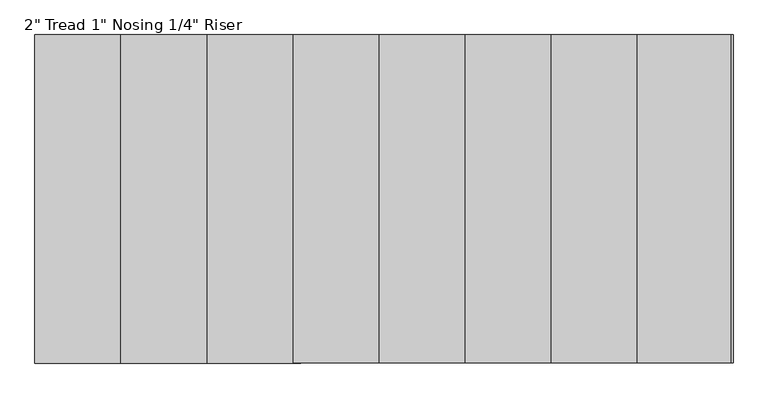
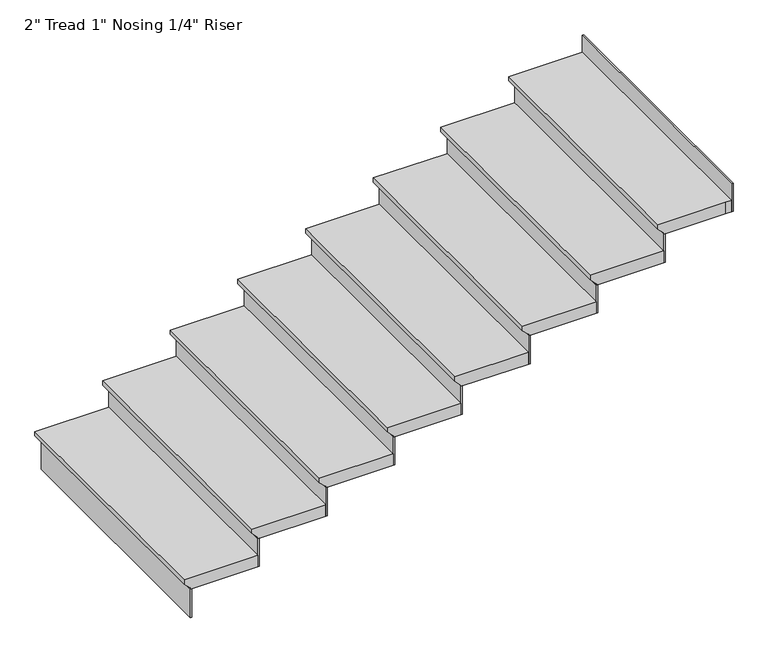
"""IFC4 building model written with IfcOpenShell, lengths in millimetres: stair flight geometry."""

from ifc_helpers import new_model, si_unit, origin, place, context, project, spatial, faceted_brep, source, transform, mapped, element, save


def stair_flight_4c000271(model_context):
    return source(origin(), model_context, "Body", "Brep", [
        faceted_brep([(663721.188677, -551651.2413841, 2328.7337838), (663721.188677, -551651.2413841, 2347.7837838), (663721.188677, -550584.4413841, 2347.7837838), (663721.188677, -550584.4413841, 2328.7337838), (663746.588677, -551651.2413841, 2303.3337838), (663746.588677, -550584.4413841, 2303.3337838), (664025.988677, -551651.2413841, 2347.7837838), (664025.988677, -550584.4413841, 2347.7837838), (663746.588677, -550584.4413841, 2296.9837838), (664025.988677, -550584.4413841, 2296.9837838), (664025.988677, -551651.2413841, 2296.9837838), (663746.588677, -551651.2413841, 2296.9837838)], [[[0, 1, 2, 3]], [[4, 0, 3, 5]], [[2, 1, 6, 7]], [[8, 9, 10, 11]], [[2, 7, 9, 8, 5, 3]], [[8, 11, 4, 5]], [[6, 1, 0, 4, 11, 10]], [[7, 6, 10, 9]]]),
        faceted_brep([(663746.588677, -551651.2413841, 2296.9837838), (663746.588677, -551651.2413841, 2173.4162162), (663752.938677, -551651.2413841, 2173.4162162), (663752.938677, -551651.2413841, 2296.9837838), (663746.588677, -550584.4413841, 2296.9837838), (663752.938677, -550584.4413841, 2296.9837838), (663752.938677, -550584.4413841, 2173.4162162), (663746.588677, -550584.4413841, 2173.4162162)], [[[0, 1, 2, 3]], [[4, 5, 6, 7]], [[1, 0, 4, 7]], [[2, 1, 7, 6]], [[3, 2, 6, 5]], [[0, 3, 5, 4]]]),
        faceted_brep([(664025.988677, -551651.2413841, 2420.5513514), (664025.988677, -551651.2413841, 2296.9837838), (664032.338677, -551651.2413841, 2296.9837838), (664032.338677, -551651.2413841, 2420.5513514), (664025.988677, -550584.4413841, 2420.5513514), (664032.338677, -550584.4413841, 2420.5513514), (664032.338677, -550584.4413841, 2296.9837838), (664025.988677, -550584.4413841, 2296.9837838)], [[[0, 1, 2, 3]], [[4, 5, 6, 7]], [[1, 0, 4, 7]], [[2, 1, 7, 6]], [[3, 2, 6, 5]], [[0, 3, 5, 4]]]),
        faceted_brep([(664000.588677, -550584.4413841, 2471.3513514), (664000.588677, -551651.2413841, 2471.3513514), (664305.388677, -551651.2413841, 2471.3513514), (664305.388677, -550584.4413841, 2471.3513514), (664025.988677, -550584.4413841, 2420.5513514), (664305.388677, -550584.4413841, 2420.5513514), (664305.388677, -551651.2413841, 2420.5513514), (664025.988677, -551651.2413841, 2420.5513514), (664025.988677, -550584.4413841, 2426.9013514), (664000.588677, -550584.4413841, 2452.3013514), (664025.988677, -551651.2413841, 2426.9013514), (664000.588677, -551651.2413841, 2452.3013514)], [[[0, 1, 2, 3]], [[4, 5, 6, 7]], [[0, 3, 5, 4, 8, 9]], [[4, 7, 10, 8]], [[2, 1, 11, 10, 7, 6]], [[3, 2, 6, 5]], [[11, 1, 0, 9]], [[10, 11, 9, 8]]]),
        faceted_brep([(664305.388677, -551651.2413841, 2544.1189189), (664305.388677, -551651.2413841, 2420.5513514), (664311.738677, -551651.2413841, 2420.5513514), (664311.738677, -551651.2413841, 2544.1189189), (664305.388677, -550584.4413841, 2544.1189189), (664311.738677, -550584.4413841, 2544.1189189), (664311.738677, -550584.4413841, 2420.5513514), (664305.388677, -550584.4413841, 2420.5513514)], [[[0, 1, 2, 3]], [[4, 5, 6, 7]], [[1, 0, 4, 7]], [[2, 1, 7, 6]], [[3, 2, 6, 5]], [[0, 3, 5, 4]]]),
        faceted_brep([(664279.988677, -550584.4413841, 2594.9189189), (664279.988677, -551651.2413841, 2594.9189189), (664584.788677, -551651.2413841, 2594.9189189), (664584.788677, -550584.4413841, 2594.9189189), (664305.388677, -550584.4413841, 2544.1189189), (664584.788677, -550584.4413841, 2544.1189189), (664584.788677, -551651.2413841, 2544.1189189), (664305.388677, -551651.2413841, 2544.1189189), (664305.388677, -550584.4413841, 2550.4689189), (664279.988677, -550584.4413841, 2575.8689189), (664305.388677, -551651.2413841, 2550.4689189), (664279.988677, -551651.2413841, 2575.8689189)], [[[0, 1, 2, 3]], [[4, 5, 6, 7]], [[0, 3, 5, 4, 8, 9]], [[4, 7, 10, 8]], [[2, 1, 11, 10, 7, 6]], [[3, 2, 6, 5]], [[11, 1, 0, 9]], [[10, 11, 9, 8]]]),
        faceted_brep([(664584.788677, -551651.2413841, 2667.6864865), (664584.788677, -551651.2413841, 2544.1189189), (664591.138677, -551651.2413841, 2544.1189189), (664591.138677, -551651.2413841, 2667.6864865), (664584.788677, -550584.4413841, 2667.6864865), (664591.138677, -550584.4413841, 2667.6864865), (664591.138677, -550584.4413841, 2544.1189189), (664584.788677, -550584.4413841, 2544.1189189)], [[[0, 1, 2, 3]], [[4, 5, 6, 7]], [[1, 0, 4, 7]], [[2, 1, 7, 6]], [[3, 2, 6, 5]], [[0, 3, 5, 4]]]),
        faceted_brep([(664559.388677, -550584.4413841, 2718.4864865), (664559.388677, -551651.2413841, 2718.4864865), (664864.188677, -551651.2413841, 2718.4864865), (664864.188677, -550584.4413841, 2718.4864865), (664584.788677, -550584.4413841, 2667.6864865), (664864.188677, -550584.4413841, 2667.6864865), (664864.188677, -551651.2413841, 2667.6864865), (664584.788677, -551651.2413841, 2667.6864865), (664584.788677, -550584.4413841, 2674.0364865), (664559.388677, -550584.4413841, 2699.4364865), (664584.788677, -551651.2413841, 2674.0364865), (664559.388677, -551651.2413841, 2699.4364865)], [[[0, 1, 2, 3]], [[4, 5, 6, 7]], [[0, 3, 5, 4, 8, 9]], [[4, 7, 10, 8]], [[2, 1, 11, 10, 7, 6]], [[3, 2, 6, 5]], [[11, 1, 0, 9]], [[10, 11, 9, 8]]]),
        faceted_brep([(664864.188677, -551651.2413841, 2791.2540541), (664864.188677, -551651.2413841, 2667.6864865), (664870.538677, -551651.2413841, 2667.6864865), (664870.538677, -551651.2413841, 2791.2540541), (664864.188677, -550584.4413841, 2791.2540541), (664870.538677, -550584.4413841, 2791.2540541), (664870.538677, -550584.4413841, 2667.6864865), (664864.188677, -550584.4413841, 2667.6864865)], [[[0, 1, 2, 3]], [[4, 5, 6, 7]], [[1, 0, 4, 7]], [[2, 1, 7, 6]], [[3, 2, 6, 5]], [[0, 3, 5, 4]]]),
        faceted_brep([(664838.788677, -550584.4413841, 2842.0540541), (664838.788677, -551651.2413841, 2842.0540541), (665143.588677, -551651.2413841, 2842.0540541), (665143.588677, -550584.4413841, 2842.0540541), (664864.188677, -550584.4413841, 2791.2540541), (665143.588677, -550584.4413841, 2791.2540541), (665143.588677, -551651.2413841, 2791.2540541), (664864.188677, -551651.2413841, 2791.2540541), (664864.188677, -550584.4413841, 2797.6040541), (664838.788677, -550584.4413841, 2823.0040541), (664864.188677, -551651.2413841, 2797.6040541), (664838.788677, -551651.2413841, 2823.0040541)], [[[0, 1, 2, 3]], [[4, 5, 6, 7]], [[0, 3, 5, 4, 8, 9]], [[4, 7, 10, 8]], [[2, 1, 11, 10, 7, 6]], [[3, 2, 6, 5]], [[11, 1, 0, 9]], [[10, 11, 9, 8]]]),
        faceted_brep([(665143.588677, -551651.2413841, 2914.8216216), (665143.588677, -551651.2413841, 2791.2540541), (665149.938677, -551651.2413841, 2791.2540541), (665149.938677, -551651.2413841, 2914.8216216), (665143.588677, -550584.4413841, 2914.8216216), (665149.938677, -550584.4413841, 2914.8216216), (665149.938677, -550584.4413841, 2791.2540541), (665143.588677, -550584.4413841, 2791.2540541)], [[[0, 1, 2, 3]], [[4, 5, 6, 7]], [[1, 0, 4, 7]], [[2, 1, 7, 6]], [[3, 2, 6, 5]], [[0, 3, 5, 4]]]),
        faceted_brep([(665118.188677, -550584.4413841, 2965.6216216), (665118.188677, -551651.2413841, 2965.6216216), (665422.988677, -551651.2413841, 2965.6216216), (665422.988677, -550584.4413841, 2965.6216216), (665143.588677, -550584.4413841, 2914.8216216), (665422.988677, -550584.4413841, 2914.8216216), (665422.988677, -551651.2413841, 2914.8216216), (665143.588677, -551651.2413841, 2914.8216216), (665143.588677, -550584.4413841, 2921.1716216), (665118.188677, -550584.4413841, 2946.5716216), (665143.588677, -551651.2413841, 2921.1716216), (665118.188677, -551651.2413841, 2946.5716216)], [[[0, 1, 2, 3]], [[4, 5, 6, 7]], [[0, 3, 5, 4, 8, 9]], [[4, 7, 10, 8]], [[2, 1, 11, 10, 7, 6]], [[3, 2, 6, 5]], [[11, 1, 0, 9]], [[10, 11, 9, 8]]]),
        faceted_brep([(665422.988677, -551651.2413841, 3038.3891892), (665422.988677, -551651.2413841, 2914.8216216), (665429.338677, -551651.2413841, 2914.8216216), (665429.338677, -551651.2413841, 3038.3891892), (665422.988677, -550584.4413841, 3038.3891892), (665429.338677, -550584.4413841, 3038.3891892), (665429.338677, -550584.4413841, 2914.8216216), (665422.988677, -550584.4413841, 2914.8216216)], [[[0, 1, 2, 3]], [[4, 5, 6, 7]], [[1, 0, 4, 7]], [[2, 1, 7, 6]], [[3, 2, 6, 5]], [[0, 3, 5, 4]]]),
        faceted_brep([(665397.588677, -550584.4413841, 3089.1891892), (665397.588677, -551651.2413841, 3089.1891892), (665702.388677, -551651.2413841, 3089.1891892), (665702.388677, -550584.4413841, 3089.1891892), (665422.988677, -550584.4413841, 3038.3891892), (665702.388677, -550584.4413841, 3038.3891892), (665702.388677, -551651.2413841, 3038.3891892), (665422.988677, -551651.2413841, 3038.3891892), (665422.988677, -550584.4413841, 3044.7391892), (665397.588677, -550584.4413841, 3070.1391892), (665422.988677, -551651.2413841, 3044.7391892), (665397.588677, -551651.2413841, 3070.1391892)], [[[0, 1, 2, 3]], [[4, 5, 6, 7]], [[0, 3, 5, 4, 8, 9]], [[4, 7, 10, 8]], [[2, 1, 11, 10, 7, 6]], [[3, 2, 6, 5]], [[11, 1, 0, 9]], [[10, 11, 9, 8]]]),
        faceted_brep([(665981.788677, -551651.2413841, 3285.5243243), (665981.788677, -551651.2413841, 3161.9567568), (665988.138677, -551651.2413841, 3161.9567568), (665988.138677, -551651.2413841, 3285.5243243), (665981.788677, -550584.4413841, 3285.5243243), (665988.138677, -550584.4413841, 3285.5243243), (665988.138677, -550584.4413841, 3161.9567568), (665981.788677, -550584.4413841, 3161.9567568)], [[[0, 1, 2, 3]], [[4, 5, 6, 7]], [[1, 0, 4, 7]], [[2, 1, 7, 6]], [[3, 2, 6, 5]], [[0, 3, 5, 4]]]),
        faceted_brep([(665702.388677, -551651.2413841, 3161.9567568), (665702.388677, -551651.2413841, 3038.3891892), (665708.738677, -551651.2413841, 3038.3891892), (665708.738677, -551651.2413841, 3161.9567568), (665702.388677, -550584.4413841, 3161.9567568), (665708.738677, -550584.4413841, 3161.9567568), (665708.738677, -550584.4413841, 3038.3891892), (665702.388677, -550584.4413841, 3038.3891892)], [[[0, 1, 2, 3]], [[4, 5, 6, 7]], [[1, 0, 4, 7]], [[2, 1, 7, 6]], [[3, 2, 6, 5]], [[0, 3, 5, 4]]]),
        faceted_brep([(665676.988677, -550584.4413841, 3212.7567568), (665676.988677, -551651.2413841, 3212.7567568), (665956.388677, -551651.2413841, 3212.7567568), (665981.788677, -551651.2413841, 3212.7567568), (665981.788677, -550584.4413841, 3212.7567568), (665702.388677, -550584.4413841, 3161.9567568), (665981.788677, -550584.4413841, 3161.9567568), (665981.788677, -551651.2413841, 3161.9567568), (665956.388677, -551651.2413841, 3161.9567568), (665702.388677, -551651.2413841, 3161.9567568), (665702.388677, -550584.4413841, 3168.3067568), (665676.988677, -550584.4413841, 3193.7067568), (665702.388677, -551651.2413841, 3168.3067568), (665676.988677, -551651.2413841, 3193.7067568)], [[[0, 1, 2, 3, 4]], [[5, 6, 7, 8, 9]], [[0, 4, 6, 5, 10, 11]], [[5, 9, 12, 10]], [[2, 1, 13, 12, 9, 8]], [[3, 2, 8, 7]], [[4, 3, 7, 6]], [[13, 1, 0, 11]], [[12, 13, 11, 10]]]),
    ])


if __name__ == "__main__":
    model = new_model("IFC4")
    model_context = context("Model", 3, world=origin())
    ifc_project = project(units=[si_unit("LENGTHUNIT", "METRE", prefix="MILLI")], contexts=[model_context])
    site = spatial("IfcSite", under=ifc_project)
    building = spatial("IfcBuilding", under=site)
    placement = place(None, origin())
    stair_flight_shape = stair_flight_4c000271(model_context)
    element("IfcStairFlight", 1, ObjectType="2\" Tread 1\" Nosing 1/4\" Riser", at=placement, inside=building, context=model_context, shape_type="MappedRepresentation", body=[
        mapped(stair_flight_shape, transform((0.0, 0.0, 0.0), x_axis=(1.0, 0.0, 0.0), y_axis=(0.0, 1.0, 0.0), z_axis=(0.0, 0.0, 1.0))),
    ])
    save(model, "model.ifc")
